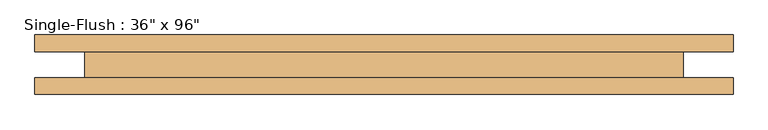
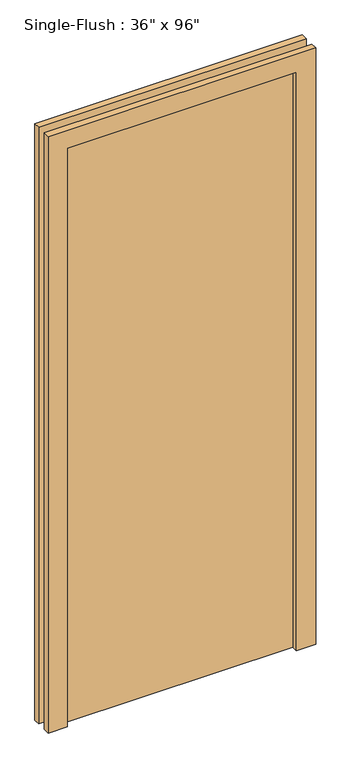
"""IFC4 building model written with IfcOpenShell, lengths in millimetres: door geometry."""

from ifc_helpers import new_model, si_unit, frame, origin, origin_with_axes, place, context, project, spatial, polyline, outline, extrude, source, transform, mapped, element, save


def door_92a4a2fc(model_context):
    return source(origin(), model_context, "Body", "SweptSolid", [
        extrude(outline(polyline([(2514.6, -533.4), (0.0, -533.4), (0.0, -457.2), (2438.4, -457.2), (2438.4, 457.2), (0.0, 457.2), (0.0, 533.4), (2514.6, 533.4), (2514.6, -533.4)])), frame((0.0, -45.39996, 0.0), z_axis=(0.0, 1.0, 0.0), x_axis=(0.0, 0.0, 1.0)), (0.0, 0.0, 1.0), 25.4),
        extrude(outline(polyline([(2514.6, 533.4), (2514.6, -533.4), (0.0, -533.4), (0.0, -457.2), (2438.4, -457.2), (2438.4, 457.2), (0.0, 457.2), (0.0, 533.4), (2514.6, 533.4)])), frame((0.0, 19.99996, 0.0), z_axis=(0.0, 1.0, 0.0), x_axis=(0.0, 0.0, 1.0)), (0.0, 0.0, 1.0), 25.4),
        extrude(outline(polyline([(457.2, 30.80004), (457.2, -19.99996), (-457.2, -19.99996), (-457.2, 30.80004), (457.2, 30.80004)])), origin_with_axes(), (0.0, 0.0, 1.0), 2438.4),
    ])


if __name__ == "__main__":
    model = new_model("IFC4")
    model_context = context("Model", 3, world=origin())
    ifc_project = project(units=[si_unit("LENGTHUNIT", "METRE", prefix="MILLI")], contexts=[model_context])
    site = spatial("IfcSite", under=ifc_project)
    building = spatial("IfcBuilding", under=site)
    placement = place(None, origin())
    door_shape = door_92a4a2fc(model_context)
    element("IfcDoor", 1, ObjectType="Single-Flush : 36\" x 96\"", at=placement, inside=building, context=model_context, shape_type="MappedRepresentation", body=[
        mapped(door_shape, transform((0.0, 0.0, 0.0), x_axis=(1.0, 0.0, 0.0), y_axis=(0.0, 1.0, 0.0), z_axis=(0.0, 0.0, 1.0))),
    ])
    save(model, "model.ifc")

# Revit data of these elements
# Type "Single-Flush : 36\" x 96\""
#   Type Mark = "32"
#   Construction Type Id = "MDOOR"
#   Assembly Code = "C1020"
#   Analytic Construction = "Metal"
#   Thickness = 0' - 2"
#   Heat Transfer Coefficient (U) = 3.7021 W/(m²·K)
#   Height = 8' - 0"
#   Trim Projection Ext = 0' - 1"
#   Trim Projection Int = 0' - 1"
#   Trim Width = 0' - 3"
#   Width = 3' - 0"
#   Door Material = Aluminum
#   Frame Material = Aluminum
#   Visual Light Transmittance = 0
#   Solar Heat Gain Coefficient = 0
#   Function = (empty or 0)
#   Wall Closure = (empty or 0)
# Element 1 (IfcDoor, "Single-Flush : 36\" x 96\"")
#   Materials on its faces: "Aluminum"
# Materials
#   "Aluminum": class "Metal", colour RGB 247 247 247, transparency 0, Description = "Aluminum 6061", Cost = 0
